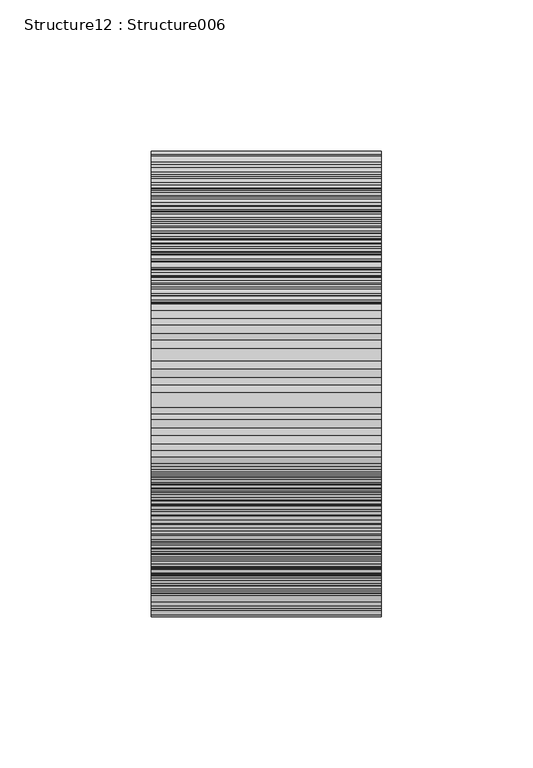
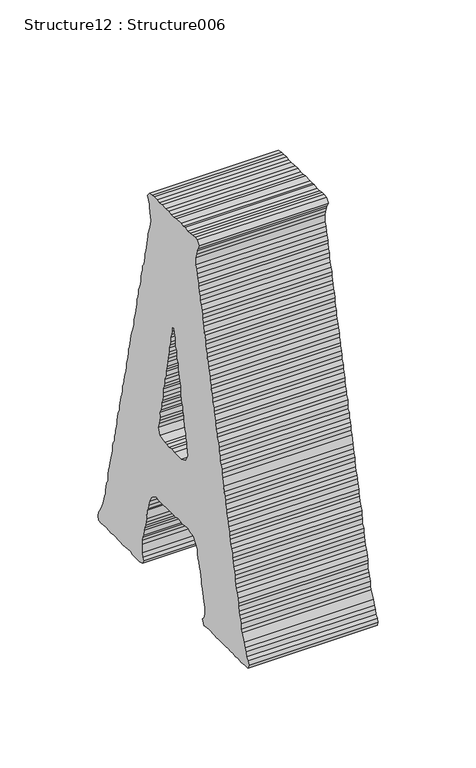
"""IFC4 building model written with IfcOpenShell, lengths in millimetres: proxy geometry, Structure12 : Structure006."""

from ifc_helpers import new_model, si_unit, frame, origin, place, context, project, spatial, polyline, outline, extrude, source, transform, mapped, element, save


def structure12_structure006_c2c7cddd(model_context):
    return source(origin(), model_context, "Body", "SweptSolid", [
        extrude(outline(polyline([(2.1653931, 0.0), (4.9551582, -1.235189), (7.1205514, -1.5528817), (9.8959144, -1.8587138), (12.3790002, -2.7770574), (14.2258535, -3.0947501), (17.0249376, -4.024107), (19.4987044, -4.024107), (22.2740675, -4.9534639), (24.4394606, -5.5651282), (27.2292257, -6.1886529), (29.3937717, -6.8011644), (31.8616083, -7.1069965), (33.7101559, -8.0363534), (36.8159193, -8.3540461), (38.9813125, -8.3540461), (41.7583699, -8.9775709), (43.3112516, -9.9069278), (46.4093904, -10.5075787), (48.2664099, -11.1311035), (50.7384823, -11.7546283), (53.207166, -11.7546283), (55.371712, -12.3781531), (58.1614771, -13.30751), (60.6428686, -14.2250064), (63.419926, -14.2250064), (65.2676265, -15.1552105), (68.3750842, -15.7787353), (70.2219375, -15.7787353), (72.7041762, -16.7080922), (75.1770958, -17.0139243), (77.9524588, -17.6374491), (80.1322541, -18.5557927), (84.4621932, -18.5557927), (86.9291825, -17.9432812), (89.4029494, -17.3197564), (91.2591217, -16.3903995), (93.7311941, -15.1552105), (96.2142799, -17.3197564), (96.5226536, -19.4851496), (96.5226536, -21.6615561), (95.9109893, -24.4386135), (95.9109893, -26.9098388), (96.5226536, -29.6979095), (96.2142799, -31.54561), (96.5226536, -33.7220165), (96.5226536, -38.664467), (95.9109893, -41.1467057), (95.9109893, -43.6179309), (96.5226536, -46.3949884), (96.2142799, -49.1949196), (96.2142799, -53.2071661), (95.9109893, -55.996084), (96.5226536, -58.1496166), (96.5226536, -60.9495479), (96.2142799, -63.1030805), (95.9109893, -65.8801379), (93.4245148, -67.7507123), (91.2591217, -66.5036627), (89.0945757, -65.8801379), (87.2375562, -65.5853192), (84.4621932, -64.9617944), (79.8094783, -64.0324375), (77.6457795, -64.6559622), (74.8687221, -65.279487), (69.9135639, -67.1271875), (68.3750842, -67.1271875), (65.5853191, -67.7507123), (63.1166354, -68.3623766), (60.3268703, -68.6800692), (57.8437845, -69.2917335), (55.371712, -70.5277697), (53.5155397, -70.5277697), (50.7384823, -70.8336018), (48.2664099, -71.4571266), (46.4093904, -72.7041762), (43.6196253, -72.7041762), (41.1467056, -73.6225198), (38.9813125, -74.234184), (36.5134759, -74.234184), (33.7101559, -74.8577088), (31.2507912, -75.7870657), (29.085398, -76.7164227), (27.2292257, -77.0341153), (24.4394606, -77.3399474), (22.2740675, -78.258291), (19.4987044, -78.258291), (17.0249376, -79.1876479), (14.8510727, -79.5053406), (12.0748624, -80.1170048), (7.7322156, -81.6588732), (4.9551582, -81.6588732), (2.7906123, -82.282398), (0.3176926, -82.9059228), (-2.4720725, -84.1411118), (-4.3282448, -84.4588045), (-6.8020116, -85.0704687), (-9.283403, -85.3881614), (-12.0604605, -86.306505), (-13.9217158, -86.9300298), (-16.7063979, -86.9300298), (-19.4826081, -87.8593867), (-21.3438635, -88.1652188), (-24.1344758, -89.0945757), (-26.5929933, -89.401255), (-29.0752319, -89.7070872), (-30.9322514, -90.330612), (-33.4136429, -91.2599689), (-36.4982268, -91.565801), (-38.9711464, -92.1893258), (-40.5240281, -93.1186827), (-43.3002383, -93.1186827), (-46.0908506, -93.7311941), (-48.2553966, -94.6605511), (-51.0409258, -95.2722153), (-52.9021812, -95.8957401), (-55.0531722, -96.5192649), (-57.5354109, -96.5192649), (-60.6327025, -97.7434406), (-63.1013862, -98.3669654), (-65.2794871, -98.684658), (-67.7524067, -98.684658), (-69.6094262, -99.2963223), (-72.6931629, -100.2256792), (-74.5501824, -100.5433719), (-77.032421, -101.4617155), (-79.8128671, -101.4617155), (-81.9782603, -102.6969045), (-84.1428062, -103.3204293), (-86.6106428, -103.3204293), (-89.386853, -103.9439541), (-92.1910202, -104.873311), (-94.3420113, -105.4858224), (-96.2032666, -106.0974867), (-98.9887958, -106.4151793), (-101.4617155, -107.3445363), (-104.2514806, -107.9680611), (-106.7193172, -107.9680611), (-108.8982652, -108.2738932), (-111.0492563, -109.4980689), (-113.8390214, -110.1215937), (-116.311941, -110.7451185), (-118.476487, -110.7451185), (-120.6503519, -111.6744754), (-125.8994818, -113.2163437), (-128.0784298, -114.1457007), (-129.9261303, -115.0750576), (-132.7116595, -116.9346186), (-134.2560694, -117.5462828), (-137.0314325, -118.4756398), (-139.2061446, -117.852115), (-139.5136711, -114.7692254), (-139.2061446, -112.9215249), (-138.8884519, -110.1215937), (-139.5136711, -107.6503684), (-139.5136711, -104.873311), (-138.8884519, -102.3910724), (-138.8884519, -100.2256792), (-139.2061446, -97.7434406), (-139.2061446, -95.589908), (-139.5136711, -92.4951579), (-139.5136711, -90.330612), (-139.2061446, -87.8593867), (-138.8884519, -85.0704687), (-139.5136711, -82.9059228), (-139.5136711, -75.7870657), (-138.8884519, -73.0100083), (-136.7374609, -71.7629588), (-134.8762055, -72.7041762), (-132.4083689, -73.3158405), (-127.1363652, -73.3158405), (-124.6634456, -73.3158405), (-122.4988996, -72.7041762), (-120.6503519, -71.7629588), (-117.5437413, -71.4571266), (-115.3791954, -70.8336018), (-113.2138022, -69.9042449), (-111.0492563, -69.2917335), (-108.5805725, -68.6800692), (-103.0145972, -68.0565444), (-101.4617155, -67.4330196), (-98.9887958, -66.5036627), (-95.8957401, -65.8801379), (-92.8018373, -64.3501301), (-90.9405819, -62.1737236), (-89.0928814, -58.7731414), (-89.7045457, -56.3019161), (-89.7045457, -51.3484522), (-89.386853, -48.2537022), (-89.386853, -41.7702305), (-89.7045457, -38.9702992), (-89.0928814, -36.8167666), (-89.386853, -34.3345279), (-89.7045457, -31.8633027), (-89.386853, -29.6979095), (-89.0928814, -26.6040066), (-89.7045457, -24.7444456), (-90.6372913, -21.0380313), (-92.4943108, -19.1793175), (-95.8957401, -16.7080922), (-98.6719504, -16.7080922), (-101.4617155, -16.0845674), (-103.0145972, -15.1552105), (-106.0991811, -14.8493783), (-107.9697554, -13.6133421), (-110.7459657, -12.9898173), (-112.6029851, -12.6839852), (-115.0759048, -12.6839852), (-117.5437413, -11.4369356), (-120.0302159, -11.1311035), (-122.4988996, -10.8252714), (-124.6634456, -9.9069278), (-127.7607372, -8.9775709), (-131.7831498, -9.283403), (-134.8762055, -10.2127599), (-136.4206154, -11.7546283), (-139.5136711, -9.9069278), (-139.2061446, -7.1069965), (-138.8884519, -4.6357712), (-138.8884519, 0.3176927), (-139.2061446, 2.7770574), (-139.2061446, 5.2601432), (-138.8884519, 7.4246892), (-139.2061446, 9.6019428), (-139.2061446, 12.6839852), (-138.8884519, 14.5435462), (-139.2061446, 17.6264358), (-138.8884519, 19.4851496), (-139.5136711, 21.9563749), (-138.8884519, 24.7563061), (-139.5136711, 27.5333635), (-139.2061446, 29.6987567), (-138.8884519, 32.1809953), (-138.8884519, 34.6403601), (-136.4206154, 35.5815775), (-134.2560694, 34.9580527), (-132.7116595, 33.405171), (-129.9261303, 32.7935068), (-128.0784298, 31.8633027), (-125.2742626, 30.6281136), (-120.6503519, 28.4627205), (-118.7797776, 27.8391957), (-115.7002768, 27.5333635), (-113.2138022, 26.9098388), (-111.0492563, 26.2981745), (-109.2015558, 25.3688176), (-106.0991811, 25.0629855), (-104.2514806, 25.0629855), (-101.4617155, 24.4386135), (-98.6719504, 23.5092566), (-96.5201121, 22.5798996), (-94.3420113, 21.9563749), (-91.565801, 21.6505427), (-89.0928814, 21.3565711), (-86.9190164, 21.0388785), (-84.7629423, 19.8028422), (-81.6563317, 19.4851496), (-79.5053406, 19.1793175), (-77.032421, 18.8734853), (-74.858556, 17.9441284), (-72.3856364, 17.0147715), (-69.6094262, 16.40226), (-68.0556973, 15.7787353), (-65.5827776, 15.7787353), (-62.7980956, 14.8493783), (-60.0074833, 14.5435462), (-58.151311, 13.9200214), (-55.6783914, 13.0016779), (-53.5223172, 12.6839852), (-50.7232331, 11.7546283), (-48.2553966, 11.7546283), (-46.0908506, 11.1311035), (-43.617931, 10.5194392), (-40.8273187, 9.8959144), (-36.1949362, 8.6598782), (-33.7220165, 8.048214), (-31.2397779, 8.048214), (-29.0752319, 7.118857), (-26.910686, 6.1895001), (-23.8125472, 6.1895001), (-21.9690826, 4.9534639), (-19.4826081, 4.9534639), (-16.7063979, 4.6476318), (-14.2250064, 3.4005822), (-12.0604605, 3.4005822), (-9.9094694, 2.1653931), (-6.8020116, 1.8477005), (-4.6366185, 1.8477005), (-1.8612554, 0.6235248), (0.0, 0.0), (2.1653931, 0.0)]), holes=[polyline([(-49.7947234, -33.0984917), (-49.7947234, -40.2173488), (-49.5007518, -42.9944062), (-50.1124161, -45.7824769), (-49.5007518, -47.9478701), (-49.7947234, -50.1132632), (-48.2553966, -54.7490344), (-44.2423029, -56.3019161), (-41.1450113, -55.6783914), (-38.9711464, -55.0667271), (-36.8150722, -54.4432023), (-33.7220165, -54.7490344), (-31.5430685, -53.5248587), (-29.0752319, -53.2071661), (-26.910686, -52.901334), (-24.7452928, -51.971977), (-22.2639014, -51.6542844), (-19.7909818, -51.6542844), (-17.0147715, -51.3484522), (-15.1535162, -50.4190953), (-12.6848324, -49.8065839), (-10.203441, -49.8065839), (-7.4221477, -48.5713948), (-4.6366185, -48.5713948), (-2.4720725, -47.6420379), (-0.6099699, -47.3243453), (2.4737668, -47.0185131), (4.9551582, -46.3949884), (7.423842, -45.7824769), (9.5892351, -45.4766448), (12.0748624, -45.4766448), (14.5435462, -44.2414557), (16.7089393, -43.9237631), (19.4987044, -43.9237631), (21.9563748, -42.9944062), (24.1353229, -42.3708814), (26.300716, -42.3708814), (26.6040066, -41.4525378), (24.1353229, -40.8408735), (21.6496955, -39.8996561), (19.1810118, -39.593824), (16.4048016, -39.593824), (14.5435462, -38.3586349), (11.7537811, -38.0409423), (9.8959144, -38.0409423), (7.423842, -36.8167666), (4.3307863, -36.4990739), (2.1653931, -36.1932418), (0.0, -35.569717), (-2.4720725, -35.2638849), (-5.2567545, -34.3345279), (-10.203441, -34.0168353), (-12.6848324, -33.4161844), (-15.1535162, -33.0984917), (-16.7063979, -32.1691348), (-19.4826081, -32.1691348), (-21.9690826, -30.9339457), (-24.4377663, -30.9339457), (-26.5929933, -30.310421), (-29.3920774, -30.0037416), (-31.2397779, -29.0862453), (-34.0159881, -29.0862453), (-36.8150722, -28.1450278), (-38.6627727, -28.1450278), (-41.1450113, -27.5333636), (-44.2423029, -26.9098388), (-47.9470229, -28.7685526), (-49.7947234, -33.0984917)])]), frame((-35624.0862846, 277190.971173, 4122.0266343), z_axis=(1.0, 0.0, 1.354250045437766e-12), x_axis=(-1.354250045437766e-12, 0.0, 1.0)), (0.0, 0.0, 1.0), 76.2),
    ])


if __name__ == "__main__":
    model = new_model("IFC4")
    model_context = context("Model", 3, world=origin())
    ifc_project = project(units=[si_unit("LENGTHUNIT", "METRE", prefix="MILLI")], contexts=[model_context])
    site = spatial("IfcSite", under=ifc_project)
    building = spatial("IfcBuilding", under=site)
    placement = place(None, origin())
    structure12_structure006_shape = structure12_structure006_c2c7cddd(model_context)
    element("IfcBuildingElementProxy", 1, Name="Structure12 : Structure006", ObjectType="Structure12 : Structure006", at=placement, inside=building, context=model_context, shape_type="MappedRepresentation", body=[
        mapped(structure12_structure006_shape, transform((0.0, 0.0, 0.0), x_axis=(1.0, 0.0, 0.0), y_axis=(0.0, 1.0, 0.0), z_axis=(0.0, 0.0, 1.0))),
    ])
    save(model, "model.ifc")

# Revit data of these elements
# Type "Structure12 : Structure006"
#   NameOverride = "Structure006"
# Element 1 (IfcBuildingElementProxy, "Structure12 : Structure006")
#   Materials on its faces: "BRUSHED ALUMINUM LETTERING"
# Materials
#   "BRUSHED ALUMINUM LETTERING": class "Unassigned", colour RGB 169 181 186, transparency 0, Cost = 0
